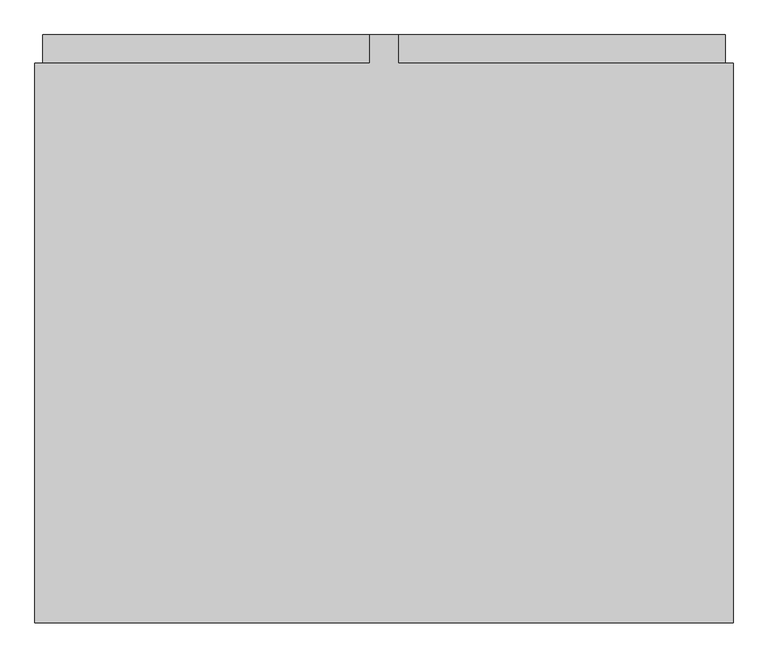
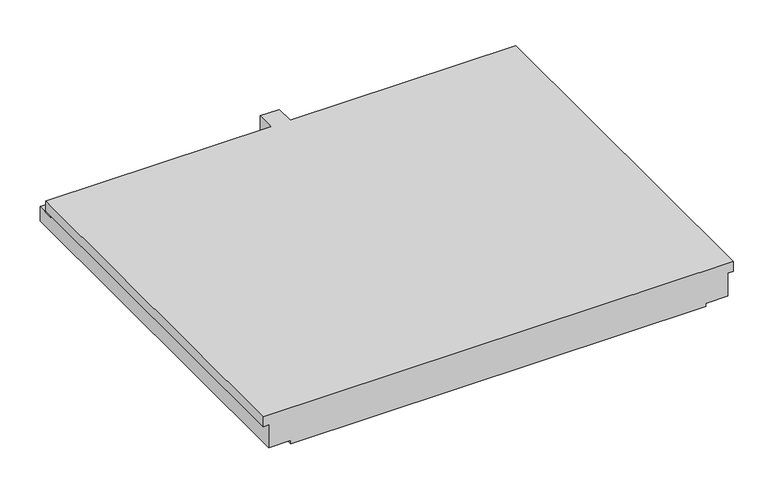
"""IFC4 building model written with IfcOpenShell, lengths in millimetres: stair geometry, NLRS_24_GM_UN_rechthoekig bordes prefab-AV_gen_rsf : prefab bordes_gen__2300x2730."""

from ifc_helpers import new_model, si_unit, origin, place, context, project, spatial, faceted_brep, source, transform, mapped, element, save


def stair_39f13373(model_context):
    return source(origin(), model_context, "Body", "Brep", [
        faceted_brep([(1365.0, 2190.0, 0.0), (1365.0, 0.0, 0.0), (1365.0, 0.0, -60.0), (1365.0, 2190.0, -60.0), (55.0, 2300.0, -110.0), (55.0, 2190.0, -110.0), (1335.0, 2190.0, -110.0), (1335.0, 2300.0, -110.0), (55.0, 2190.0, 0.0), (1335.0, 2190.0, -60.0), (55.0, 2300.0, 0.0), (-55.0, 2300.0, 0.0), (-55.0, 2300.0, -110.0), (-55.0, 2190.0, -110.0), (-55.0, 2190.0, 0.0), (-1365.0, 0.0, 0.0), (-1365.0, 2190.0, 0.0), (-1365.0, 2190.0, -60.0), (-1365.0, 0.0, -60.0), (-1335.0, 2300.0, -110.0), (1335.0, 2300.0, -200.0), (1205.0, 2300.0, -200.0), (1205.0, 2300.0, -220.0), (-1205.0, 2300.0, -220.0), (-1205.0, 2300.0, -200.0), (-1335.0, 2300.0, -200.0), (-1335.0, 2190.0, -110.0), (-1335.0, 2190.0, -60.0), (-1335.0, 0.0, -60.0), (-1335.0, 0.0, -200.0), (-1205.0, 0.0, -200.0), (-1205.0, 0.0, -220.0), (1205.0, 0.0, -220.0), (1205.0, 0.0, -200.0), (1335.0, 0.0, -200.0), (1335.0, 0.0, -60.0)], [[[0, 1, 2, 3]], [[4, 5, 6, 7]], [[8, 0, 3, 9, 6, 5]], [[10, 8, 5, 4]], [[11, 12, 13, 14]], [[15, 16, 17, 18]], [[19, 12, 11, 10, 4, 7, 20, 21, 22, 23, 24, 25]], [[12, 19, 26, 13]], [[16, 14, 13, 26, 27, 17]], [[16, 15, 1, 0, 8, 10, 11, 14]], [[15, 18, 28, 29, 30, 31, 32, 33, 34, 35, 2, 1]], [[31, 23, 22, 32]], [[27, 28, 18, 17]], [[25, 29, 28, 27, 26, 19]], [[29, 25, 24, 30]], [[30, 24, 23, 31]], [[35, 9, 3, 2]], [[34, 20, 7, 6, 9, 35]], [[20, 34, 33, 21]], [[21, 33, 32, 22]]]),
    ])


if __name__ == "__main__":
    model = new_model("IFC4")
    model_context = context("Model", 3, world=origin())
    ifc_project = project(units=[si_unit("LENGTHUNIT", "METRE", prefix="MILLI")], contexts=[model_context])
    site = spatial("IfcSite", under=ifc_project)
    building = spatial("IfcBuilding", under=site)
    placement = place(None, origin())
    stair_shape = stair_39f13373(model_context)
    element("IfcStair", 1, ObjectType="NLRS_24_GM_UN_rechthoekig bordes prefab-AV_gen_rsf : prefab bordes_gen__2300x2730", at=placement, inside=building, context=model_context, shape_type="MappedRepresentation", body=[
        mapped(stair_shape, transform((0.0, 0.0, 0.0), x_axis=(1.0, 0.0, 0.0), y_axis=(0.0, 1.0, 0.0), z_axis=(0.0, 0.0, 1.0))),
    ])
    save(model, "model.ifc")

# Revit data of these elements
# Type "NLRS_24_GM_UN_rechthoekig bordes prefab-AV_gen_rsf : prefab bordes_gen__2300x2730"
#   IfcExportAs = "IfcStair"
#   Type Comments = " "
#   Model = " "
#   Manufacturer = " "
#   Description = "rechthoekig bordes prefab\r\n1930x4395"
#   Assembly Code = "24.15"
#   Width = 2730 mm
#   Thickness = 220 mm
#   Perimeter = 10060 mm
#   NLRS_C_lengte_02 = 1310 mm
#   NLRS_C_lengte_01 = 1310 mm
#   NLRS_C_hoogte_02 = 110 mm
#   NLRS_C_hoogte_01 = 110 mm
#   NLRS_C_diepte_04 = 2300 mm
#   NLRS_C_diepte_03 = 2300 mm
#   NLRS_C_diepte_02 = 110 mm
#   NLRS_C_diepte_01 = 110 mm
#   Length = 2300 mm
#   Default Elevation = 1219.2 mm
#   Area = 6.279 m²
#   NLRS_C_materiaal = NLRS_f2_beton prefab_gen_rsf
#   Keynote = ""
# Element 1 (IfcStair, "NLRS_24_GM_UN_rechthoekig bordes prefab-AV_gen_rsf : prefab bordes_gen__2300x2730")
#   Materials on its faces: "NLRS_f2_beton prefab_gen_rsf"
# Materials
#   "NLRS_f2_beton prefab_gen_rsf": class "F - Niet gebakken kunststeen", colour RGB 129 133 118, transparency 0, Keynote = "f2", Manufacturer = "Revit Standards Foundation", URL = "www.revitstandards.org", Description = "beton prefab", Cost = 0
